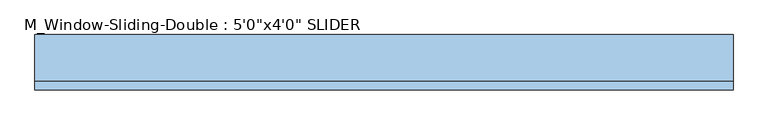
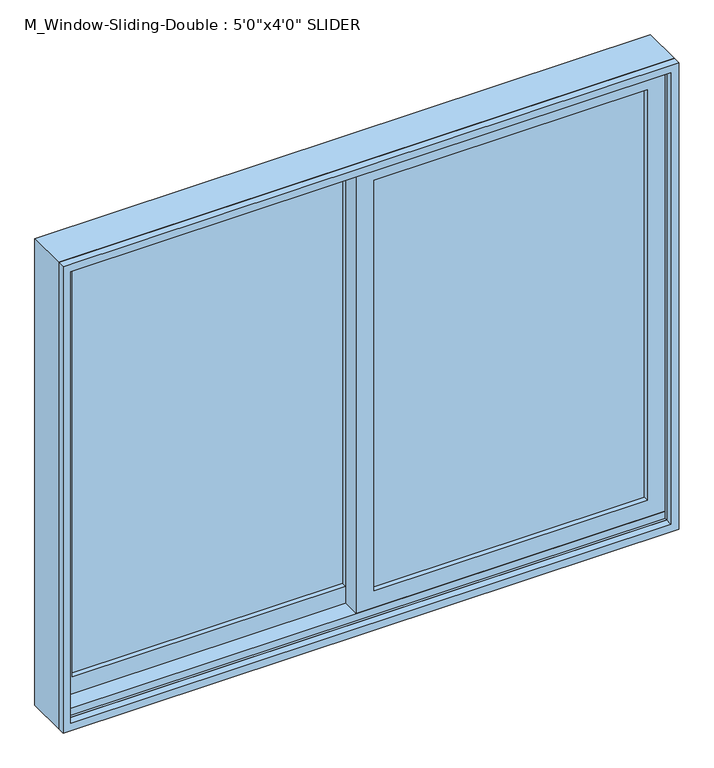
"""IFC4 building model written with IfcOpenShell, lengths in millimetres: window geometry."""

from ifc_helpers import new_model, si_unit, frame, origin, place, context, project, spatial, polyline, outline, extrude, faceted_brep, source, transform, mapped, element, save


def window_17206027(model_context):
    return source(origin(), model_context, "Body", "SolidModel", [
        faceted_brep([(-762.0, -35.56, 900.0), (-762.0, 66.04, 900.0), (762.0, 66.04, 900.0), (762.0, -35.56, 900.0), (-721.0778905, 66.04, 2078.2778905), (-721.0778905, 59.69, 2078.2778905), (-721.0778905, 59.69, 919.05), (-721.0778905, 66.04, 919.05), (721.0778905, 59.69, 2078.2778905), (721.0778905, 59.69, 919.05), (742.95, 59.69, 919.05), (742.95, 59.69, 2100.15), (-742.95, 59.69, 2100.15), (-742.95, 59.69, 919.05), (-742.95, -35.56, 2100.15), (-742.95, -35.56, 919.05), (-742.95, -29.21, 919.05), (-742.95, -29.21, 938.1), (-742.95, 15.24, 938.1), (-742.95, 15.24, 919.05), (762.0, -35.56, 2119.2), (-762.0, -35.56, 2119.2), (742.95, -35.56, 2100.15), (742.95, -35.56, 919.05), (-762.0, 66.04, 2119.2), (762.0, 66.04, 2119.2), (721.0778905, 66.04, 919.05), (721.0778905, 66.04, 2078.2778905), (742.95, 15.24, 919.05), (742.95, 15.24, 938.1), (742.95, -29.21, 938.1), (742.95, -29.21, 919.05)], [[[0, 1, 2, 3]], [[4, 5, 6, 7]], [[5, 8, 9, 10, 11, 12, 13, 6]], [[12, 14, 15, 16, 17, 18, 19, 13]], [[0, 3, 20, 21], [22, 23, 15, 14]], [[24, 1, 0, 21]], [[2, 1, 24, 25], [4, 7, 26, 27]], [[5, 4, 27, 8]], [[12, 11, 22, 14]], [[21, 20, 25, 24]], [[8, 27, 26, 9]], [[22, 11, 10, 28, 29, 30, 31, 23]], [[20, 3, 2, 25]], [[26, 7, 6, 13, 19, 28, 10, 9]], [[28, 19, 18, 29]], [[29, 18, 17, 30]], [[30, 17, 16, 31]], [[15, 23, 31, 16]]]),
        extrude(outline(polyline([(2119.2, -762.0), (900.0, -762.0), (900.0, 762.0), (2119.2, 762.0), (2119.2, -762.0)]), holes=[polyline([(2100.15, 742.95), (919.05, 742.95), (919.05, -742.95), (2100.15, -742.95), (2100.15, 742.95)])]), frame((0.0, -54.61, 0.0), z_axis=(0.0, 1.0, 0.0), x_axis=(0.0, 0.0, 1.0)), (0.0, 0.0, 1.0), 19.05),
        extrude(outline(polyline([(698.5, 2.54), (698.5, -3.81), (22.225, -3.81), (22.225, 2.54), (698.5, 2.54)])), frame((0.0, 0.0, 982.55), z_axis=(0.0, 0.0, 1.0), x_axis=(1.0, 0.0, 0.0)), (0.0, 0.0, 1.0), 1073.15),
        extrude(outline(polyline([(698.5, -10.16), (698.5, -16.51), (22.225, -16.51), (22.225, -10.16), (698.5, -10.16)])), frame((0.0, 0.0, 982.55), z_axis=(0.0, 0.0, 1.0), x_axis=(1.0, 0.0, 0.0)), (0.0, 0.0, 1.0), 1073.15),
        extrude(outline(polyline([(-22.225, 46.99), (-22.225, 40.64), (-698.5, 40.64), (-698.5, 46.99), (-22.225, 46.99)])), frame((0.0, 0.0, 982.55), z_axis=(0.0, 0.0, 1.0), x_axis=(1.0, 0.0, 0.0)), (0.0, 0.0, 1.0), 1073.15),
        extrude(outline(polyline([(-22.225, 34.29), (-22.225, 27.94), (-698.5, 27.94), (-698.5, 34.29), (-22.225, 34.29)])), frame((0.0, 0.0, 982.55), z_axis=(0.0, 0.0, 1.0), x_axis=(1.0, 0.0, 0.0)), (0.0, 0.0, 1.0), 1073.15),
        extrude(outline(polyline([(919.05, -742.95), (919.05, 22.225), (2100.15, 22.225), (2100.15, -742.95), (919.05, -742.95)]), holes=[polyline([(2055.7, -22.225), (982.55, -22.225), (982.55, -698.5), (2055.7, -698.5), (2055.7, -22.225)])]), frame((0.0, 15.24, 0.0), z_axis=(0.0, 1.0, 0.0), x_axis=(0.0, 0.0, 1.0)), (0.0, 0.0, 1.0), 44.45),
        extrude(outline(polyline([(938.1, 742.95), (2100.15, 742.95), (2100.15, -22.225), (938.1, -22.225), (938.1, 742.95)]), holes=[polyline([(982.55, 22.225), (2055.7, 22.225), (2055.7, 698.5), (982.55, 698.5), (982.55, 22.225)])]), frame((0.0, -29.21, 0.0), z_axis=(0.0, 1.0, 0.0), x_axis=(0.0, 0.0, 1.0)), (0.0, 0.0, 1.0), 44.45),
    ])


if __name__ == "__main__":
    model = new_model("IFC4")
    model_context = context("Model", 3, world=origin())
    ifc_project = project(units=[si_unit("LENGTHUNIT", "METRE", prefix="MILLI")], contexts=[model_context])
    site = spatial("IfcSite", under=ifc_project)
    building = spatial("IfcBuilding", under=site)
    placement = place(None, origin())
    window_shape = window_17206027(model_context)
    element("IfcWindow", 1, ObjectType="M_Window-Sliding-Double : 5'0\"x4'0\" SLIDER", at=placement, inside=building, context=model_context, shape_type="MappedRepresentation", body=[
        mapped(window_shape, transform((0.0, 0.0, 0.0), x_axis=(1.0, 0.0, 0.0), y_axis=(0.0, 1.0, 0.0), z_axis=(0.0, 0.0, 1.0))),
    ])
    save(model, "model.ifc")

# Revit data of these elements
# Type "M_Window-Sliding-Double : 5'0\"x4'0\" SLIDER"
#   Type Mark = "6"
#   Fire Rating = "0.5h"
#   Assembly Code = "B2020100"
#   Analytic Construction = "Double glazing - domestic"
#   Window Inset [instance default] = 0' - 0"
#   Wall Thickness [instance default] = 0' - 5.90551"
#   Visual Light Transmittance = 0.81
#   Thermal Resistance (R) = 1.8146 (h·ft²·°F)/BTU
#   Solar Heat Gain Coefficient = 0.76
#   Muntin Width = 2' - 2 5/8"
#   Muntin Height = 3' - 6 1/4"
#   Interior Wall Closure [instance default] = 0' - 2.65551"
#   Heat Transfer Coefficient (U) = 0.5511 BTU/(h·ft²·°F)
#   Frame Extension [instance default] = 0' - 0 1/4"
#   Exterior Wall Closure [instance default] = 0' - 1 1/4"
#   Rough Width = 5' - 0.59055"
#   Rough Height = 4' - 0.59055"
#   Height = 4' - 0"
#   Extension Jamb [instance default] = 0' - 2.65551"
#   Default Sill Height = 2' - 11.43307"
#   Width = 5' - 0"
#   Interior Trim Visibility [instance default] = yes
#   Indicator Visibility [instance default] = yes
#   Exterior Trim Visibility [instance default] = yes
#   Muntin Visibility = yes
#   Extension Jamb Visibility [instance default] = yes
#   Muntin Pattern = M_Muntin Pattern_2x2 : M_Muntin Pattern_2x2
#   Interior Trim Material = Wood - Stained
#   Interior Trim = M_Trim-Window-Interior-Flat : Picture Frame
#   Interior Frame Material = Wood - Stained
#   Glass Panel Material = Glass
#   Exterior Trim Material = Clad - White
#   Exterior Trim = M_Trim-Window-Exterior-Flat : with Sill
#   Exterior Frame Material = Clad - White
#   Wall Closure = (empty or 0)
# Element 1 (IfcWindow, "M_Window-Sliding-Double : 5'0\"x4'0\" SLIDER")
#   Wall Thickness = 0' - 4"
#   Extension Jamb = 0' - 0 3/4"
#   Materials on its faces: "Wood - Stained", "Glass", "Clad - White"
# Materials
#   "Wood - Stained": class "Wood", colour RGB 224 178 126, transparency 0, Cost = 0
#   "Glass": class "Glass", colour RGB 0 128 192, transparency 0.75, Description = "Soda Lime Glass", Cost = 0
#   "Clad - White": class "Wood", colour RGB 242 242 238, transparency 0, Cost = 0
